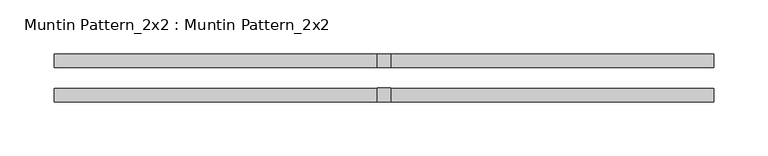
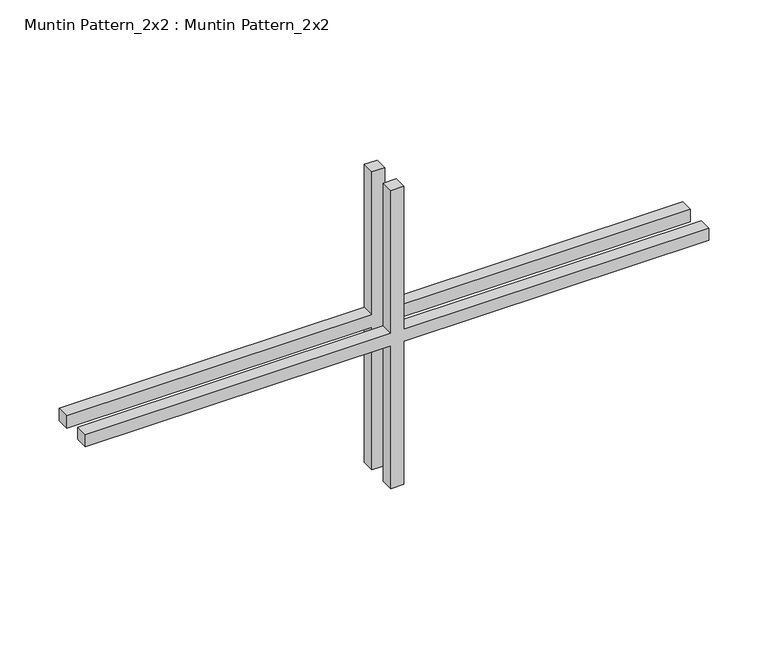
"""IFC4 building model written with IfcOpenShell, lengths in millimetres: proxy geometry, Muntin Pattern_2x2 : Muntin Pattern_2x2."""

from ifc_helpers import new_model, si_unit, frame, origin, place, context, project, spatial, polyline, outline, extrude, source, transform, mapped, element, save


def muntin_pattern_2x2_muntin_pattern_2x2_a77e86ff(model_context):
    return source(origin(), model_context, "Body", "SweptSolid", [
        extrude(outline(polyline([(160.3375, -6.35), (160.3375, -304.8), (147.6375, -304.8), (147.6375, -6.35), (0.0, -6.35), (0.0, 6.35), (147.6375, 6.35), (147.6375, 304.8), (160.3375, 304.8), (160.3375, 6.35), (307.975, 6.35), (307.975, -6.35), (160.3375, -6.35)])), frame((0.0, 9.525, 0.0), z_axis=(0.0, 1.0, 0.0), x_axis=(0.0, 0.0, 1.0)), (0.0, 0.0, 1.0), 12.7),
        extrude(outline(polyline([(160.3375, -6.35), (160.3375, -304.8), (147.6375, -304.8), (147.6375, -6.35), (0.0, -6.35), (0.0, 6.35), (147.6375, 6.35), (147.6375, 304.8), (160.3375, 304.8), (160.3375, 6.35), (307.975, 6.35), (307.975, -6.35), (160.3375, -6.35)])), frame((0.0, -22.225, 0.0), z_axis=(0.0, 1.0, 0.0), x_axis=(0.0, 0.0, 1.0)), (0.0, 0.0, 1.0), 12.7),
    ])


if __name__ == "__main__":
    model = new_model("IFC4")
    model_context = context("Model", 3, world=origin())
    ifc_project = project(units=[si_unit("LENGTHUNIT", "METRE", prefix="MILLI")], contexts=[model_context])
    site = spatial("IfcSite", under=ifc_project)
    building = spatial("IfcBuilding", under=site)
    placement = place(None, origin())
    muntin_pattern_2x2_muntin_pattern_2x2_shape = muntin_pattern_2x2_muntin_pattern_2x2_a77e86ff(model_context)
    element("IfcBuildingElementProxy", 1, Name="Muntin Pattern_2x2 : Muntin Pattern_2x2", ObjectType="Muntin Pattern_2x2 : Muntin Pattern_2x2", at=placement, inside=building, context=model_context, shape_type="MappedRepresentation", body=[
        mapped(muntin_pattern_2x2_muntin_pattern_2x2_shape, transform((0.0, 0.0, 0.0), x_axis=(1.0, 0.0, 0.0), y_axis=(0.0, 1.0, 0.0), z_axis=(0.0, 0.0, 1.0))),
    ])
    save(model, "model.ifc")

# Revit data of these elements
# Type "Muntin Pattern_2x2 : Muntin Pattern_2x2"
#   Width [instance default] = 4' - 0"
#   Thickness = 0' - 0 1/2"
#   Height [instance default] = 4' - 0"
#   Distance = 0' - 0 3/4"
#   Interior Material [instance default] = none
#   Exterior Material [instance default] = none
# Element 1 (IfcBuildingElementProxy, "Muntin Pattern_2x2 : Muntin Pattern_2x2")
#   Width = 2' - 0"
#   Height = 1' - 0 1/8"
#   Interior Material = Wood - Stained
#   Exterior Material = Clad - White
#   Materials on its faces: "Clad - White", "Wood - Stained"
# Materials
#   "Clad - White": class "Wood", colour RGB 242 242 238, transparency 0, Cost = 0
#   "Wood - Stained": class "Wood", colour RGB 224 178 126, transparency 0, Cost = 0
